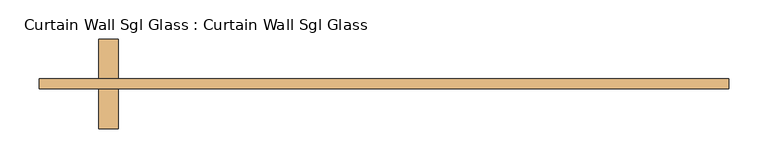
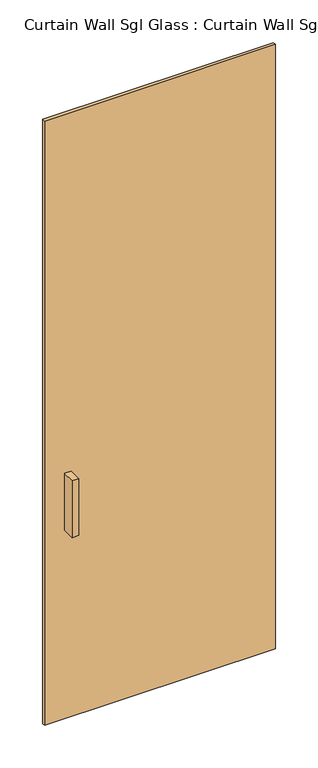
"""IFC4 building model written with IfcOpenShell, lengths in millimetres: door geometry, Curtain Wall Sgl Glass : Curtain Wall Sgl Glass."""

from ifc_helpers import new_model, si_unit, frame, origin, origin_with_axes, place, context, project, spatial, polyline, outline, extrude, source, transform, mapped, element, save


def curtain_wall_sgl_glass_curtain_wall_sgl_glass_1c17b042(model_context):
    return source(origin(), model_context, "Body", "SweptSolid", [
        extrude(outline(polyline([(-339.725, 12.7), (-339.725, -38.1), (-365.125, -38.1), (-365.125, 12.7), (-339.725, 12.7)])), frame((0.0, 0.0, 762.0), z_axis=(0.0, 0.0, 1.0), x_axis=(1.0, 0.0, 0.0)), (0.0, 0.0, 1.0), 228.6),
        extrude(outline(polyline([(-365.125, -101.6), (-365.125, -50.8), (-339.725, -50.8), (-339.725, -101.6), (-365.125, -101.6)])), frame((0.0, 0.0, 762.0), z_axis=(0.0, 0.0, 1.0), x_axis=(1.0, 0.0, 0.0)), (0.0, 0.0, 1.0), 228.6),
        extrude(outline(polyline([(441.325, -50.8), (-441.325, -50.8), (-441.325, -38.1), (441.325, -38.1), (441.325, -50.8)])), origin_with_axes(), (0.0, 0.0, 1.0), 2438.4),
    ])


if __name__ == "__main__":
    model = new_model("IFC4")
    model_context = context("Model", 3, world=origin())
    ifc_project = project(units=[si_unit("LENGTHUNIT", "METRE", prefix="MILLI")], contexts=[model_context])
    site = spatial("IfcSite", under=ifc_project)
    building = spatial("IfcBuilding", under=site)
    placement = place(None, origin())
    curtain_wall_sgl_glass_curtain_wall_sgl_glass_shape = curtain_wall_sgl_glass_curtain_wall_sgl_glass_1c17b042(model_context)
    element("IfcDoor", 1, ObjectType="Curtain Wall Sgl Glass : Curtain Wall Sgl Glass", at=placement, inside=building, context=model_context, shape_type="MappedRepresentation", body=[
        mapped(curtain_wall_sgl_glass_curtain_wall_sgl_glass_shape, transform((0.0, 0.0, 0.0), x_axis=(1.0, 0.0, 0.0), y_axis=(0.0, 1.0, 0.0), z_axis=(0.0, 0.0, 1.0))),
    ])
    save(model, "model.ifc")

# Revit data of these elements
# Type "Curtain Wall Sgl Glass : Curtain Wall Sgl Glass"
#   Type Mark = "8"
#   Assembly Code = "B2030100"
#   Thickness = 50.8 mm
#   Offset = 50.8 mm
#   Define Thermal Properties by = 0
#   Function = 1
#   Handle Material = Metal - Aluminum
#   Glazing Material = Glass
# Element 1 (IfcDoor, "Curtain Wall Sgl Glass : Curtain Wall Sgl Glass")
#   Materials on its faces: "Metal - Aluminum", "Glass"
# Materials
#   "Metal - Aluminum": class "Metal", colour RGB 247 247 247, transparency 0, Cost = 0
#   "Glass": class "Glass", colour RGB 154 182 205, transparency 0.5, Cost = 0
